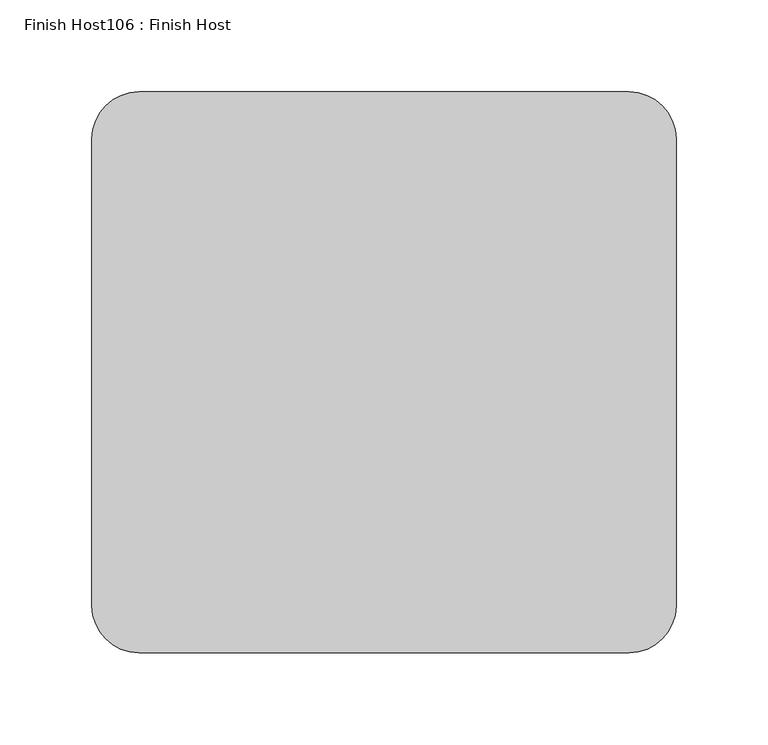
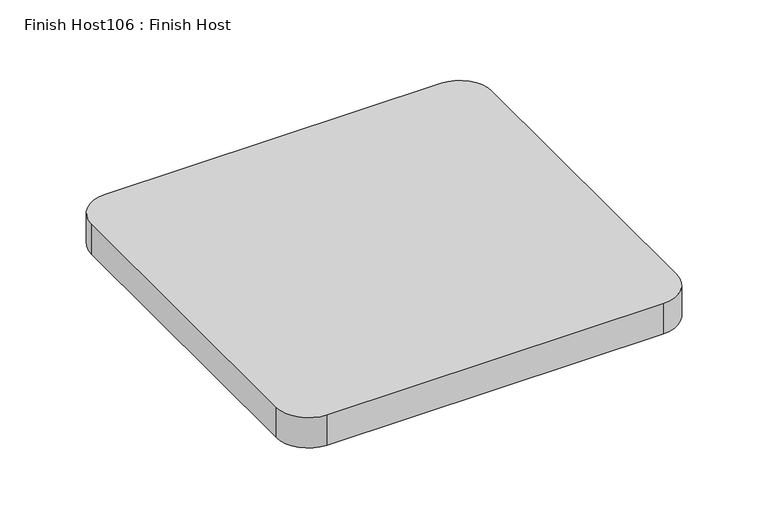
"""IFC4 building model written with IfcOpenShell, lengths in millimetres: proxy geometry, Finish Host106 : Finish Host."""

from ifc_helpers import new_model, si_unit, point, frame_2d, origin, origin_with_axes, place, context, project, spatial, polyline, circle_curve, trimmed, segment, composite_curve, outline, extrude, source, transform, mapped, element, save


def finish_host106_finish_host_d881f509(model_context):
    return source(origin(), model_context, "Body", "SweptSolid", [
        extrude(outline(composite_curve([segment(polyline([(-797.1842816, 4229.4760864), (-797.1842816, 4483.4760864)]), True, "CONTINUOUS"), segment(trimmed(circle_curve(frame_2d((-771.7842816, 4483.4760864)), 25.4), [point((-797.1842816, 4483.4760864))], [point((-771.7842816, 4508.8760864))], False, "CARTESIAN"), True, "CONTINUOUS"), segment(polyline([(-771.7842816, 4508.8760864), (-505.0842816, 4508.8760864)]), True, "CONTINUOUS"), segment(trimmed(circle_curve(frame_2d((-505.0842816, 4483.4760864)), 25.4), [point((-505.0842816, 4508.8760864))], [point((-479.6842816, 4483.4760864))], False, "CARTESIAN"), True, "CONTINUOUS"), segment(polyline([(-479.6842816, 4483.4760864), (-479.6842816, 4229.4760864)]), True, "CONTINUOUS"), segment(trimmed(circle_curve(frame_2d((-505.0842816, 4229.4760864)), 25.4), [point((-479.6842816, 4229.4760864))], [point((-505.0842816, 4204.0760864))], False, "CARTESIAN"), True, "CONTINUOUS"), segment(polyline([(-505.0842816, 4204.0760864), (-771.7842816, 4204.0760864)]), True, "CONTINUOUS"), segment(trimmed(circle_curve(frame_2d((-771.7842816, 4229.4760864)), 25.4), [point((-771.7842816, 4204.0760864))], [point((-797.1842816, 4229.4760864))], False, "CARTESIAN"), True, "CONTINUOUS")], self_intersect=False)), origin_with_axes(), (0.0, 0.0, 1.0), 25.4),
    ])


if __name__ == "__main__":
    model = new_model("IFC4")
    model_context = context("Model", 3, world=origin())
    ifc_project = project(units=[si_unit("LENGTHUNIT", "METRE", prefix="MILLI")], contexts=[model_context])
    site = spatial("IfcSite", under=ifc_project)
    building = spatial("IfcBuilding", under=site)
    placement = place(None, origin())
    finish_host106_finish_host_shape = finish_host106_finish_host_d881f509(model_context)
    element("IfcBuildingElementProxy", 1, Name="Finish Host106 : Finish Host", ObjectType="Finish Host106 : Finish Host", at=placement, inside=building, context=model_context, shape_type="MappedRepresentation", body=[
        mapped(finish_host106_finish_host_shape, transform((0.0, 0.0, 0.0), x_axis=(1.0, 0.0, 0.0), y_axis=(0.0, 1.0, 0.0), z_axis=(0.0, 0.0, 1.0))),
    ])
    save(model, "model.ifc")

# Revit data of these elements
# Type "Finish Host106 : Finish Host"
#   Panel Material = Fabric - Teknion - T100 - Topology - Ceramic
# Element 1 (IfcBuildingElementProxy, "Finish Host106 : Finish Host")
#   Materials on its faces: "Fabric - Teknion - T100 - Topology - Ceramic"
# Materials
#   "Fabric - Teknion - T100 - Topology - Ceramic": class "Fabric", colour RGB 67 65 62, transparency 0, Model = "T100", Manufacturer = "Teknion Studio", URL = "http://www.teknionstudio.com/", Description = "Ceramic Topology", Cost = 0
